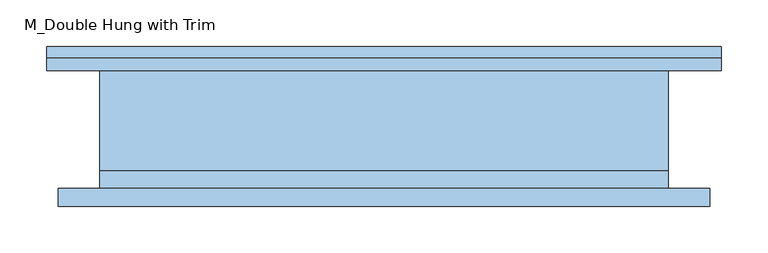
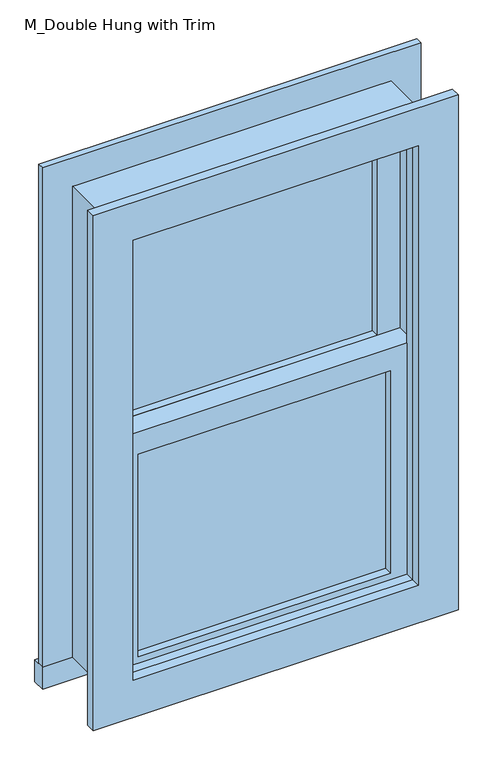
"""IFC4 building model written with IfcOpenShell, lengths in millimetres: window geometry, M_Double Hung with Trim."""

from ifc_helpers import new_model, si_unit, frame, origin, place, context, project, spatial, polyline, outline, extrude, source, transform, mapped, element, save


def m_double_hung_with_trim_8e83f439(model_context):
    return source(origin(), model_context, "Body", "SweptSolid", [
        extrude(outline(polyline([(-241.3, -15.825), (241.3, -15.825), (241.3, -28.525), (-241.3, -28.525), (-241.3, -15.825)])), frame((0.0, 0.0, 628.65), z_axis=(0.0, 0.0, 1.0), x_axis=(1.0, 0.0, 0.0)), (0.0, 0.0, 1.0), 409.575),
        extrude(outline(polyline([(1082.675, -285.75), (584.2, -285.75), (584.2, 285.75), (1082.675, 285.75), (1082.675, -285.75)]), holes=[polyline([(1038.225, -241.3), (1038.225, 241.3), (628.65, 241.3), (628.65, -241.3), (1038.225, -241.3)])]), frame((0.0, -44.4, 0.0), z_axis=(0.0, 1.0, 0.0), x_axis=(0.0, 0.0, 1.0)), (0.0, 0.0, 1.0), 44.45),
        extrude(outline(polyline([(-361.95, 89.2), (361.95, 89.2), (361.95, 63.5), (-361.95, 63.5), (-361.95, 89.2)])), frame((0.0, 0.0, 539.75), z_axis=(0.0, 0.0, 1.0), x_axis=(1.0, 0.0, 0.0)), (0.0, 0.0, 1.0), 44.45),
        extrude(outline(polyline([(1593.85, -361.95), (539.75, -361.95), (539.75, 361.95), (1593.85, 361.95), (1593.85, -361.95)]), holes=[polyline([(1517.65, -285.75), (1517.65, 285.75), (584.2, 285.75), (584.2, -285.75), (1517.65, -285.75)])]), frame((0.0, 63.5, 0.0), z_axis=(0.0, 1.0, 0.0), x_axis=(0.0, 0.0, 1.0)), (0.0, 0.0, 1.0), 13.0),
        extrude(outline(polyline([(1581.15, 349.25), (1581.15, -349.25), (539.75, -349.25), (539.75, 349.25), (1581.15, 349.25)]), holes=[polyline([(1504.95, 273.05), (615.95, 273.05), (615.95, -273.05), (1504.95, -273.05), (1504.95, 273.05)])]), frame((0.0, -82.5, 0.0), z_axis=(0.0, 1.0, 0.0), x_axis=(0.0, 0.0, 1.0)), (0.0, 0.0, 1.0), 19.0),
        extrude(outline(polyline([(241.3, 15.925), (-241.3, 15.925), (-241.3, 28.625), (241.3, 28.625), (241.3, 15.925)])), frame((0.0, 0.0, 1082.675), z_axis=(0.0, 0.0, 1.0), x_axis=(1.0, 0.0, 0.0)), (0.0, 0.0, 1.0), 390.525),
        extrude(outline(polyline([(1517.65, -285.75), (1038.225, -285.75), (1038.225, 285.75), (1517.65, 285.75), (1517.65, -285.75)]), holes=[polyline([(1473.2, -241.3), (1473.2, 241.3), (1082.675, 241.3), (1082.675, -241.3), (1473.2, -241.3)])]), frame((0.0, 0.05, 0.0), z_axis=(0.0, 1.0, 0.0), x_axis=(0.0, 0.0, 1.0)), (0.0, 0.0, 1.0), 44.45),
        extrude(outline(polyline([(1536.7, -304.8), (584.2, -304.8), (584.2, 304.8), (1536.7, 304.8), (1536.7, -304.8)]), holes=[polyline([(1504.95, -273.05), (1504.95, 273.05), (615.95, 273.05), (615.95, -273.05), (1504.95, -273.05)])]), frame((0.0, -63.5, 0.0), z_axis=(0.0, 1.0, 0.0), x_axis=(0.0, 0.0, 1.0)), (0.0, 0.0, 1.0), 19.1),
        extrude(outline(polyline([(1536.7, 304.8), (1536.7, -304.8), (584.2, -304.8), (584.2, 304.8), (1536.7, 304.8)]), holes=[polyline([(1517.65, 285.75), (603.25, 285.75), (603.25, -285.75), (1517.65, -285.75), (1517.65, 285.75)])]), frame((0.0, -44.4, 0.0), z_axis=(0.0, 1.0, 0.0), x_axis=(0.0, 0.0, 1.0)), (0.0, 0.0, 1.0), 107.9),
    ])


if __name__ == "__main__":
    model = new_model("IFC4")
    model_context = context("Model", 3, world=origin())
    ifc_project = project(units=[si_unit("LENGTHUNIT", "METRE", prefix="MILLI")], contexts=[model_context])
    site = spatial("IfcSite", under=ifc_project)
    building = spatial("IfcBuilding", under=site)
    placement = place(None, origin())
    m_double_hung_with_trim_shape = m_double_hung_with_trim_8e83f439(model_context)
    element("IfcWindow", 1, ObjectType="M_Double Hung with Trim : 2'  0\" x 3'  1 1/2\"", at=placement, inside=building, context=model_context, shape_type="MappedRepresentation", body=[
        mapped(m_double_hung_with_trim_shape, transform((0.0, 0.0, 0.0), x_axis=(1.0, 0.0, 0.0), y_axis=(0.0, 1.0, 0.0), z_axis=(0.0, 0.0, 1.0))),
    ])
    save(model, "model.ifc")

# Revit data of these elements
# Type "M_Double Hung with Trim : 2'  0\" x 3'  1 1/2\""
#   Type Mark = "71"
#   Construction Type Id = "GSP4R"
#   Analytic Construction = "1/8 in Pilkington single glazing"
#   Visual Light Transmittance = 0.9
#   Thermal Resistance (R) = 0.271106 (m²·K)/W
#   Solar Heat Gain Coefficient = 0.78
#   Heat Transfer Coefficient (U) = 3.6886 W/(m²·K)
#   Height = 3' - 1 1/2"
#   Default Sill Height = 1' - 11"
#   Trim Projection - Ext. = 0' - 0.51181"
#   Trim Projection - Int. = 0' - 0.74803"
#   Trim Width - Exterior = 0' - 3"
#   Trim Width - Interior = 0' - 3"
#   Width = 2' - 0"
#   Window Inset = 0' - 0.74803"
#   Glass Pane Material = EXISTING WINDOW
#   Sash = Trim
#   Trim Exterior Material = Trim
#   Trim Interior Material = Trim
#   Wall Closure = (empty or 0)
# Element 1 (IfcWindow, "M_Double Hung with Trim : 2'  0\" x 3'  1 1/2\"")
#   Materials on its faces: "Trim", "EXISTING WINDOW"
# Materials
#   "EXISTING WINDOW": class "Glass", colour RGB 218 227 224, transparency 0.85, Description = "Soda Lime Glass", Cost = 0
#   "Trim": class "Wood", colour RGB 250 251 245, transparency 0, Cost = 0
